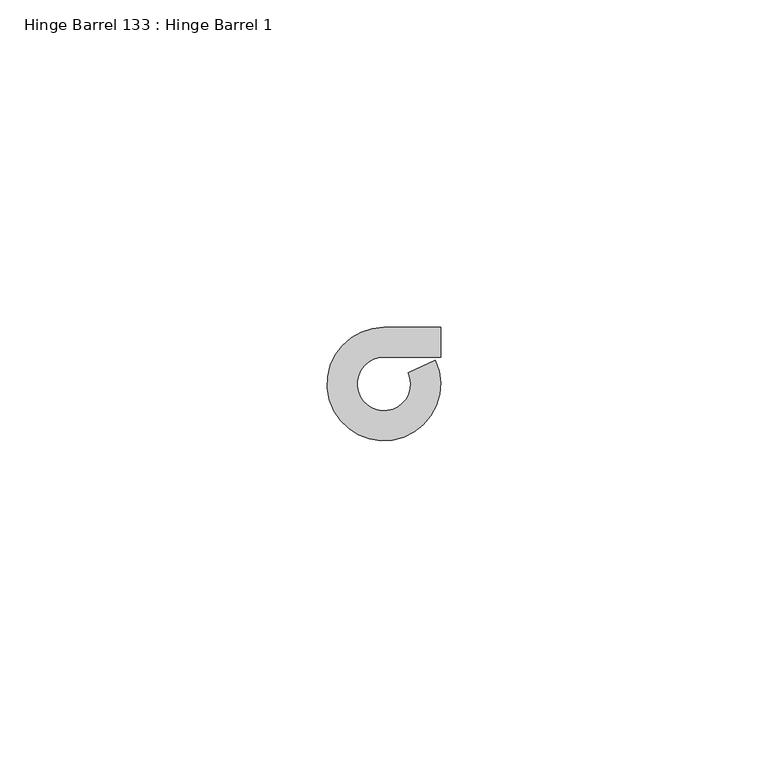
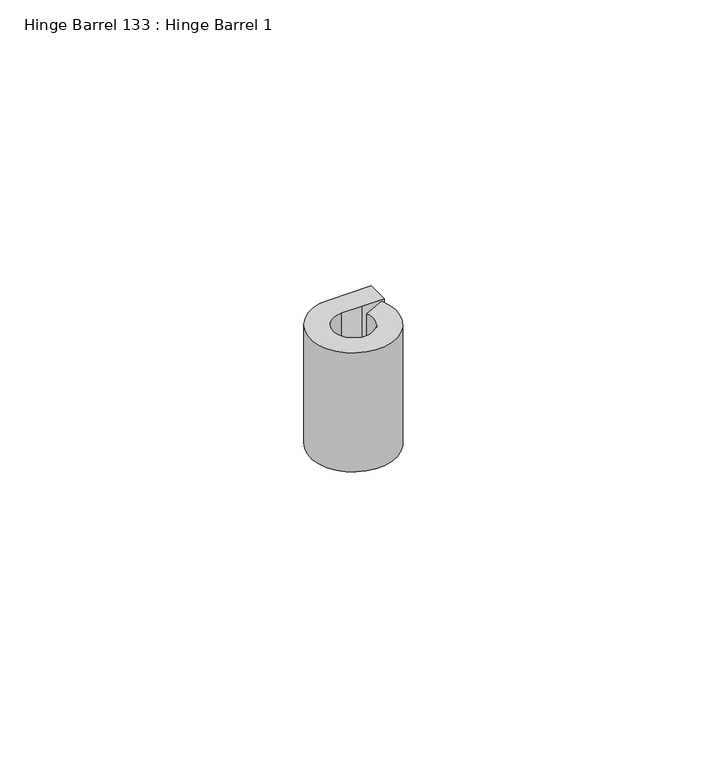
"""IFC4 building model written with IfcOpenShell, lengths in millimetres: proxy geometry, Hinge Barrel 133 : Hinge Barrel 1."""

from ifc_helpers import new_model, si_unit, point, frame, frame_2d, origin, place, context, project, spatial, polyline, circle_curve, trimmed, segment, composite_curve, outline, extrude, source, transform, mapped, element, save


def hinge_barrel_133_hinge_barrel_1_56b842ac(model_context):
    return source(origin(), model_context, "Body", "SweptSolid", [
        extrude(outline(composite_curve([segment(polyline([(587323.2214739, -536306.2758841), (587319.1320739, -536306.2758841)]), True, "CONTINUOUS"), segment(trimmed(circle_curve(frame_2d((587319.1320739, -536310.3652841)), 4.0894), [point((587319.1320739, -536306.2758841))], [point((587322.8436736, -536308.6485371))], True, "CARTESIAN"), True, "CONTINUOUS"), segment(polyline([(587322.8436736, -536308.6485371), (587326.986084, -536306.7325249)]), True, "CONTINUOUS"), segment(trimmed(circle_curve(frame_2d((587319.1320739, -536310.3652841)), 8.6534625), [point((587326.986084, -536306.7325249))], [point((587319.1320739, -536301.7118216))], False, "CARTESIAN"), True, "CONTINUOUS"), segment(polyline([(587319.1320739, -536301.7118216), (587327.7934739, -536301.7118216), (587327.7934739, -536306.2758841), (587323.2214739, -536306.2758841)]), True, "CONTINUOUS")], self_intersect=False)), frame((0.0, 0.0, 1936.75), z_axis=(0.0, 0.0, 1.0), x_axis=(1.0, 0.0, 0.0)), (0.0, 0.0, 1.0), 25.4),
    ])


if __name__ == "__main__":
    model = new_model("IFC4")
    model_context = context("Model", 3, world=origin())
    ifc_project = project(units=[si_unit("LENGTHUNIT", "METRE", prefix="MILLI")], contexts=[model_context])
    site = spatial("IfcSite", under=ifc_project)
    building = spatial("IfcBuilding", under=site)
    placement = place(None, origin())
    hinge_barrel_133_hinge_barrel_1_shape = hinge_barrel_133_hinge_barrel_1_56b842ac(model_context)
    element("IfcBuildingElementProxy", 1, Name="Hinge Barrel 133 : Hinge Barrel 1", ObjectType="Hinge Barrel 133 : Hinge Barrel 1", at=placement, inside=building, context=model_context, shape_type="MappedRepresentation", body=[
        mapped(hinge_barrel_133_hinge_barrel_1_shape, transform((0.0, 0.0, 0.0), x_axis=(1.0, 0.0, 0.0), y_axis=(0.0, 1.0, 0.0), z_axis=(0.0, 0.0, 1.0))),
    ])
    save(model, "model.ifc")

# Revit data of these elements
# Element 1 (IfcBuildingElementProxy, "Hinge Barrel 133 : Hinge Barrel 1")
#   Materials on its faces: "6\"X6\" WELD-ON STL BUTT HINGE"
# Materials
#   "6\"X6\" WELD-ON STL BUTT HINGE": class "Metal", colour RGB 189 187 185, transparency 0, Description = "Carbon steel", Cost = 0
